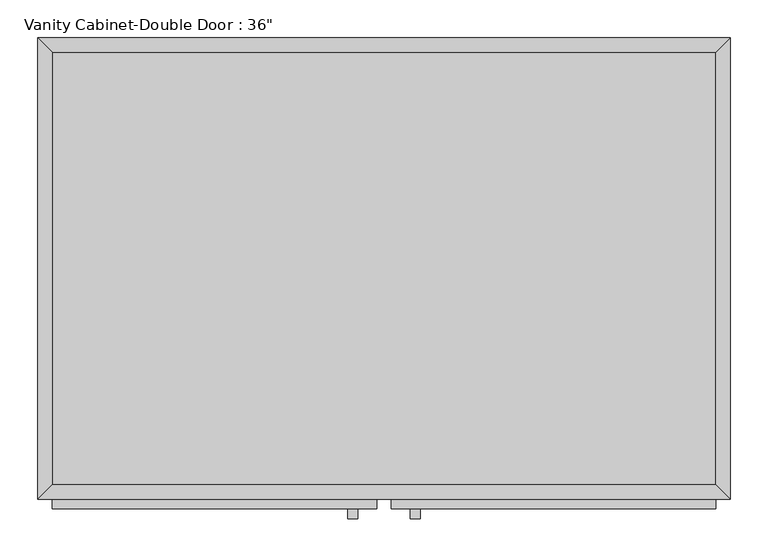
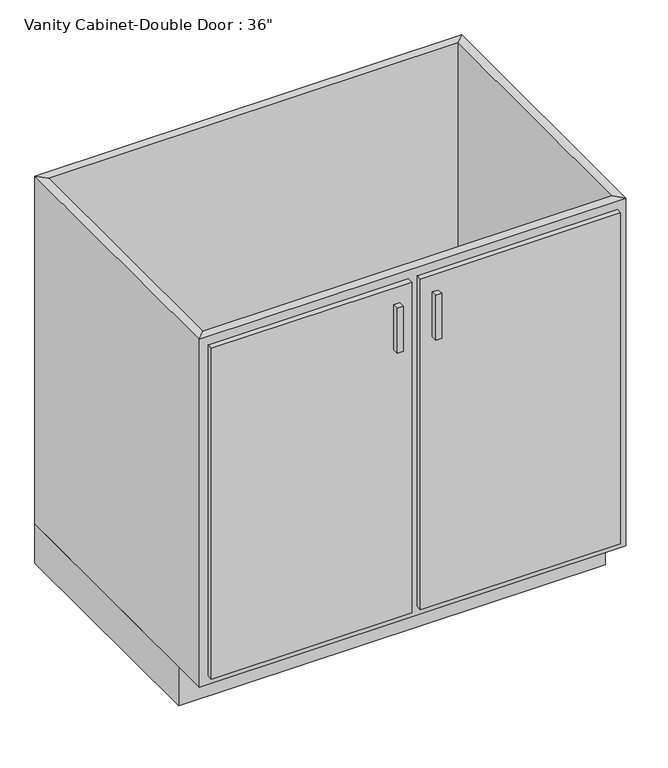
"""IFC4 building model written with IfcOpenShell, lengths in millimetres: furniture geometry."""

import ifcopenshell
import ifcopenshell.guid

model = None  # the IFC model being written
_history = None  # IfcOwnerHistory: only IFC2X3 demands one
_inside = {}  # id of a spatial element -> (the spatial element, [elements in it])
_under = {}  # id of a project, library or spatial element -> (it, [spatial elements below it])
_declared = {}  # id of a project -> (the project, [libraries it declares])
_typed = {}  # id of a type object -> (the type object, [elements of that type])
_made_of = {}  # id of a material, layer set ... -> (it, [elements and type objects made of it])


def new_model(schema):
    """Start an empty IFC model of exactly this schema.

    Asked for "IFC4X3", IfcOpenShell would pick the latest addendum, in which some entities
    have other attributes; the version numbers below select the first issue.
    IFC2X3 requires an IfcOwnerHistory on every rooted entity: one is made here for all.
    """
    global model, _history
    if schema == "IFC4X3":
        model = ifcopenshell.file(schema_version=(4, 3, 0, 0))
    else:
        model = ifcopenshell.file(schema=schema)
    _inside.clear()
    _under.clear()
    _declared.clear()
    _typed.clear()
    _made_of.clear()
    _history = None
    if model.schema == "IFC2X3":
        org = make("IfcOrganization", Name="unknown")
        user = make(
            "IfcPersonAndOrganization",
            ThePerson=make("IfcPerson", FamilyName="unknown"),
            TheOrganization=org,
        )
        app = make(
            "IfcApplication",
            ApplicationDeveloper=org,
            Version="unknown",
            ApplicationFullName="unknown",
            ApplicationIdentifier="unknown",
        )
        _history = make(
            "IfcOwnerHistory",
            OwningUser=user,
            OwningApplication=app,
            ChangeAction="ADDED",
            CreationDate=0,
        )
    return model


def make(cls, **values):
    """One entity of the class cls with the attributes given. An attribute that is None is left unset."""
    return model.create_entity(
        cls, **{name: value for name, value in values.items() if value is not None}
    )


def rooted(cls, **values):
    """An entity with a GlobalId (a new one), such as an element, a storey or a relation."""
    return make(cls, GlobalId=ifcopenshell.guid.new(), OwnerHistory=_history, **values)


def si_unit(unit_type, name, prefix=None):
    """IfcSIUnit, for example si_unit("LENGTHUNIT", "METRE", prefix="MILLI")."""
    return make("IfcSIUnit", UnitType=unit_type, Prefix=prefix, Name=name)


def assignment(units):
    """IfcUnitAssignment: the units of a project."""
    return None if units is None else make("IfcUnitAssignment", Units=units)


def point(xyz):
    """IfcCartesianPoint."""
    return None if xyz is None else make("IfcCartesianPoint", Coordinates=xyz)


def direction(xyz):
    """IfcDirection."""
    return None if xyz is None else make("IfcDirection", DirectionRatios=xyz)


def frame(location, z_axis=None, x_axis=None):
    """IfcAxis2Placement3D, a coordinate frame: its origin and axes. An axis left out is left unset."""
    return make(
        "IfcAxis2Placement3D",
        Location=point(location),
        Axis=direction(z_axis),
        RefDirection=direction(x_axis),
    )


def origin():
    """The frame at (0, 0, 0) with its axes left unset."""
    return frame((0.0, 0.0, 0.0))


def origin_with_axes():
    """The frame at (0, 0, 0) with the z axis (0, 0, 1) and the x axis (1, 0, 0) written out."""
    return frame((0.0, 0.0, 0.0), z_axis=(0.0, 0.0, 1.0), x_axis=(1.0, 0.0, 0.0))


def place(relative_to, where):
    """IfcLocalPlacement: puts the frame where relative to a parent placement (None: the world)."""
    return make(
        "IfcLocalPlacement", PlacementRelTo=relative_to, RelativePlacement=where
    )


def context(
    kind, dimensions, precision=None, world=None, true_north=None, identifier=None
):
    """IfcGeometricRepresentationContext, for example the 3D "Model" context."""
    return make(
        "IfcGeometricRepresentationContext",
        ContextIdentifier=identifier,
        ContextType=kind,
        CoordinateSpaceDimension=dimensions,
        Precision=precision,
        WorldCoordinateSystem=world,
        TrueNorth=true_north,
    )


def project(units=None, contexts=None):
    """IfcProject with its units and contexts."""
    return rooted(
        "IfcProject",
        Name="project",
        RepresentationContexts=contexts,
        UnitsInContext=assignment(units),
    )


def spatial(cls, under=None, at=None, **own):
    """A site, building, storey or space (cls), placed at a placement, below another one or the project."""
    s = rooted(cls, ObjectPlacement=at, **own)
    if under is not None:
        _under.setdefault(under.id(), (under, []))[1].append(s)
    return s


def polyline(points):
    """IfcPolyline through the points."""
    return make("IfcPolyline", Points=[point(p) for p in points])


def outline(outer, holes=None, kind="AREA"):
    """IfcArbitraryClosedProfileDef: a profile drawn as a closed curve; with holes, ...WithVoids."""
    if holes is None:
        return make("IfcArbitraryClosedProfileDef", ProfileType=kind, OuterCurve=outer)
    return make(
        "IfcArbitraryProfileDefWithVoids",
        ProfileType=kind,
        OuterCurve=outer,
        InnerCurves=holes,
    )


def extrude(swept, where, along, depth):
    """IfcExtrudedAreaSolid: the profile swept, set in the frame where, extruded along a direction by depth."""
    return make(
        "IfcExtrudedAreaSolid",
        SweptArea=swept,
        Position=where,
        ExtrudedDirection=direction(along),
        Depth=depth,
    )


def faces_of(points, faces, orient=None, outer=None):
    """IfcFace entities. A face is a list of loops; a loop is a list of indices into points, from 0.

    orient and outer hold one flag for each loop. By default every Orientation is true, the
    first loop of a face is its IfcFaceOuterBound and the others are IfcFaceBound.
    """
    made = []
    for i, loops in enumerate(faces):
        bounds = []
        for j, loop in enumerate(loops):
            is_outer = j == 0 if outer is None else outer[i][j]
            bounds.append(
                make(
                    "IfcFaceOuterBound" if is_outer else "IfcFaceBound",
                    Bound=make("IfcPolyLoop", Polygon=[points[k] for k in loop]),
                    Orientation=True if orient is None else orient[i][j],
                )
            )
        made.append(make("IfcFace", Bounds=bounds))
    return made


def faceted_brep(points, faces, orient=None, outer=None, voids=None):
    """IfcFacetedBrep: a solid bounded by flat faces; with voids (closed shells), ...WithVoids."""
    shared = [point(p) for p in points]
    hull = make("IfcClosedShell", CfsFaces=faces_of(shared, faces, orient, outer))
    if voids is None:
        return make("IfcFacetedBrep", Outer=hull)
    return make(
        "IfcFacetedBrepWithVoids",
        Outer=hull,
        Voids=[
            make(cls, CfsFaces=faces_of(shared, fs, o, b)) for cls, fs, o, b in voids
        ],
    )


def shape(context_of_items, identifier, shape_type, items):
    """IfcShapeRepresentation: the items that make up one representation, for example the "Body"."""
    return make(
        "IfcShapeRepresentation",
        ContextOfItems=context_of_items,
        RepresentationIdentifier=identifier,
        RepresentationType=shape_type,
        Items=items,
    )


def source(mapping_origin, context_of_items, identifier, shape_type, items):
    """IfcRepresentationMap: a shape defined once, which mapped items show again and again."""
    return make(
        "IfcRepresentationMap",
        MappingOrigin=mapping_origin,
        MappedRepresentation=shape(context_of_items, identifier, shape_type, items),
    )


def transform(
    local_origin,
    x_axis=None,
    y_axis=None,
    z_axis=None,
    scale=None,
    scale2=None,
    scale3=None,
    uniform=True,
):
    """IfcCartesianTransformationOperator3D, or its non-uniform kind. x_axis, y_axis, z_axis: its Axis1, 2, 3."""
    if uniform:
        return make(
            "IfcCartesianTransformationOperator3D",
            Axis1=direction(x_axis),
            Axis2=direction(y_axis),
            LocalOrigin=point(local_origin),
            Scale=scale,
            Axis3=direction(z_axis),
        )
    return make(
        "IfcCartesianTransformationOperator3DnonUniform",
        Axis1=direction(x_axis),
        Axis2=direction(y_axis),
        LocalOrigin=point(local_origin),
        Scale=scale,
        Axis3=direction(z_axis),
        Scale2=scale2,
        Scale3=scale3,
    )


def mapped(mapping_source, mapping_target):
    """IfcMappedItem: shows the shape of a source again, moved by a transform."""
    return make(
        "IfcMappedItem", MappingSource=mapping_source, MappingTarget=mapping_target
    )


def made_of(thing, what):
    """Note that an element or type object is made of a material, layer set ...; save() writes the relation."""
    if what is not None:
        _made_of.setdefault(what.id(), (what, []))[1].append(thing)
    return thing


def element(
    cls,
    number,
    at=None,
    inside=None,
    cuts=None,
    type_object=None,
    material=None,
    context=None,
    identifier="Body",
    shape_type=None,
    held_by="IfcProductDefinitionShape",
    body=None,
    shapes=None,
    **own,
):
    """One element of the class cls, such as IfcWall. Its Tag is "e" and its number.

    at: its placement. inside: the storey or other place that contains it. cuts: it is an
    opening in that element (IfcRelVoidsElement). A single representation is given by context,
    identifier, shape_type and body (its items); several are given by shapes. held_by: the class
    of the entity that holds the representations. save() writes the other relations.
    """
    e = rooted(cls, Tag="e%d" % number, ObjectPlacement=at, **own)
    if body is not None:
        shapes = [shape(context, identifier, shape_type, body)]
    if shapes is not None:
        e.Representation = make(held_by, Representations=shapes)
    if inside is not None:
        _inside.setdefault(inside.id(), (inside, []))[1].append(e)
    if cuts is not None:
        rooted(
            "IfcRelVoidsElement", RelatingBuildingElement=cuts, RelatedOpeningElement=e
        )
    if type_object is not None:
        _typed.setdefault(type_object.id(), (type_object, []))[1].append(e)
    return made_of(e, material)


def aggregate(whole, parts):
    """IfcRelAggregates: a whole, such as a stair, and the parts it consists of."""
    return rooted("IfcRelAggregates", RelatingObject=whole, RelatedObjects=parts)


def save(model, path):
    """Write the relations noted so far, then the file.

    IfcRelAggregates (storeys below a building ...), IfcRelContainedInSpatialStructure (elements
    in a storey), IfcRelDefinesByType, IfcRelAssociatesMaterial and IfcRelDeclares: one each for
    every whole, place, type object, material and project.
    """
    for whole, parts in _under.values():
        aggregate(whole, parts)
    for where, things in _inside.values():
        rooted(
            "IfcRelContainedInSpatialStructure",
            RelatedElements=things,
            RelatingStructure=where,
        )
    for kind, things in _typed.values():
        rooted("IfcRelDefinesByType", RelatedObjects=things, RelatingType=kind)
    for what, things in _made_of.values():
        rooted("IfcRelAssociatesMaterial", RelatedObjects=things, RelatingMaterial=what)
    for by, libraries in _declared.values():
        rooted("IfcRelDeclares", RelatingContext=by, RelatedDefinitions=libraries)
    model.write(path)


def furniture_aeada037(model_context):
    return source(origin(), model_context, "Body", "SolidModel", [
        extrude(outline(polyline([(456.8877049, -19.05), (456.8877049, -590.55), (-419.4122951, -590.55), (-419.4122951, -19.05), (456.8877049, -19.05)])), frame((0.0, 0.0, 88.9), z_axis=(0.0, 0.0, 1.0), x_axis=(1.0, 0.0, 0.0)), (0.0, 0.0, 1.0), 19.05),
        faceted_brep([(456.8877049, -590.55, 876.3), (456.8877049, -590.55, 88.9), (-419.4122951, -590.55, 88.9), (-419.4122951, -590.55, 876.3), (475.9377049, -609.6, 876.3), (-438.4622951, -609.6, 876.3), (475.9377049, -609.6, 88.9), (-438.4622951, -609.6, 88.9), (-419.4122951, -19.05, 88.9), (-419.4122951, -19.05, 876.3), (-438.4622951, 0.0, 876.3), (-438.4622951, 0.0, 88.9), (456.8877049, -19.05, 88.9), (456.8877049, -19.05, 876.3), (475.9377049, 0.0, 876.3), (475.9377049, 0.0, 88.9)], [[[0, 1, 2, 3]], [[4, 0, 3, 5]], [[6, 4, 5, 7]], [[1, 6, 7, 2]], [[3, 2, 8, 9]], [[5, 3, 9, 10]], [[7, 5, 10, 11]], [[2, 7, 11, 8]], [[9, 8, 12, 13]], [[10, 9, 13, 14]], [[11, 10, 14, 15]], [[8, 11, 15, 12]], [[13, 12, 1, 0]], [[14, 13, 0, 4]], [[15, 14, 4, 6]], [[12, 15, 6, 1]]]),
        extrude(outline(polyline([(475.9377049, 0.0), (475.9377049, -533.4), (-438.4622951, -533.4), (-438.4622951, 0.0), (475.9377049, 0.0)])), origin_with_axes(), (0.0, 0.0, 1.0), 88.9),
        extrude(outline(polyline([(-16.1872951, -635.0), (-28.8872951, -635.0), (-28.8872951, -622.3), (-16.1872951, -622.3), (-16.1872951, -635.0)])), frame((0.0, 0.0, 717.55), z_axis=(0.0, 0.0, 1.0), x_axis=(1.0, 0.0, 0.0)), (0.0, 0.0, 1.0), 101.6),
        extrude(outline(polyline([(66.3627049, -635.0), (53.6627049, -635.0), (53.6627049, -622.3), (66.3627049, -622.3), (66.3627049, -635.0)])), frame((0.0, 0.0, 717.55), z_axis=(0.0, 0.0, 1.0), x_axis=(1.0, 0.0, 0.0)), (0.0, 0.0, 1.0), 101.6),
        extrude(outline(polyline([(9.2127049, -622.3), (-419.4122951, -622.3), (-419.4122951, -609.6), (9.2127049, -609.6), (9.2127049, -622.3)])), frame((0.0, 0.0, 107.95), z_axis=(0.0, 0.0, 1.0), x_axis=(1.0, 0.0, 0.0)), (0.0, 0.0, 1.0), 749.3),
        extrude(outline(polyline([(456.8877049, -622.3), (28.2627049, -622.3), (28.2627049, -609.6), (456.8877049, -609.6), (456.8877049, -622.3)])), frame((0.0, 0.0, 107.95), z_axis=(0.0, 0.0, 1.0), x_axis=(1.0, 0.0, 0.0)), (0.0, 0.0, 1.0), 749.3),
    ])


if __name__ == "__main__":
    model = new_model("IFC4")
    model_context = context("Model", 3, world=origin())
    ifc_project = project(units=[si_unit("LENGTHUNIT", "METRE", prefix="MILLI")], contexts=[model_context])
    site = spatial("IfcSite", under=ifc_project)
    building = spatial("IfcBuilding", under=site)
    placement = place(None, origin())
    furniture_shape = furniture_aeada037(model_context)
    element("IfcFurniture", 1, ObjectType="Vanity Cabinet-Double Door : 36\"", at=placement, inside=building, context=model_context, shape_type="MappedRepresentation", body=[
        mapped(furniture_shape, transform((0.0, 0.0, 0.0), x_axis=(1.0, 0.0, 0.0), y_axis=(0.0, 1.0, 0.0), z_axis=(0.0, 0.0, 1.0))),
    ])
    save(model, "model.ifc")

# Revit data of these elements
# Type "Vanity Cabinet-Double Door : 36\""
#   Finish = "Cabinetry"
#   Assembly Code = "C1030410"
#   Depth = 2' - 0"
#   Height = 2' - 10 1/2"
#   Toe Depth = 0' - 3"
#   Toe Height = 0' - 3 1/2"
#   Width = 3' - 0"
#   Cabinet Material = Cabinets
#   Door/Drawer Material = Cabinets
#   Handle Material = Cabinets - Handles
# Element 1 (IfcFurniture, "Vanity Cabinet-Double Door : 36\"")
#   Materials on its faces: "Cabinets", "Cabinets - Handles"
# Materials
#   "Cabinets": class "Paint", colour RGB 249 249 249, transparency 0
#   "Cabinets - Handles": class "Metal", colour RGB 57 57 57, transparency 0
